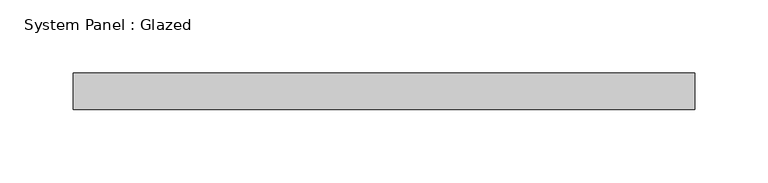
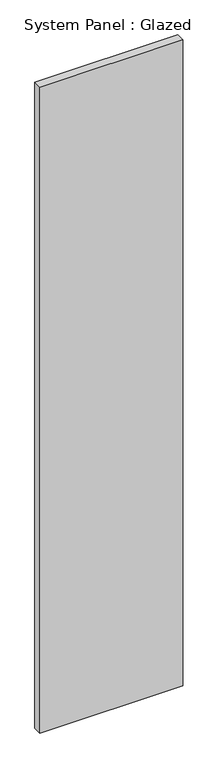
"""IFC4 building model written with IfcOpenShell, lengths in millimetres: plate geometry, System Panel : Glazed."""

from ifc_helpers import new_model, si_unit, origin, origin_with_axes, place, context, project, spatial, polyline, outline, extrude, source, transform, mapped, element, save


def system_panel_glazed_248dfa94(model_context):
    return source(origin(), model_context, "Body", "SweptSolid", [
        extrude(outline(polyline([(212.5000001, 24.5), (-212.5000001, 24.5), (-212.5000001, 49.5), (212.5000001, 49.5), (212.5000001, 24.5)])), origin_with_axes(), (0.0, 0.0, 1.0), 2030.4462072),
    ])


if __name__ == "__main__":
    model = new_model("IFC4")
    model_context = context("Model", 3, world=origin())
    ifc_project = project(units=[si_unit("LENGTHUNIT", "METRE", prefix="MILLI")], contexts=[model_context])
    site = spatial("IfcSite", under=ifc_project)
    building = spatial("IfcBuilding", under=site)
    placement = place(None, origin())
    system_panel_glazed_shape = system_panel_glazed_248dfa94(model_context)
    element("IfcPlate", 1, ObjectType="System Panel : Glazed", at=placement, inside=building, context=model_context, shape_type="MappedRepresentation", body=[
        mapped(system_panel_glazed_shape, transform((0.0, 0.0, 0.0), x_axis=(1.0, 0.0, 0.0), y_axis=(0.0, 1.0, 0.0), z_axis=(0.0, 0.0, 1.0))),
    ])
    save(model, "model.ifc")

# Revit data of these elements
# Type "System Panel : Glazed"
#   Construction Type Id = "GSP4R"
#   Analytic Construction = "1/8 in Pilkington single glazing"
#   Visual Light Transmittance = 0.9
#   Solar Heat Gain Coefficient = 0.86
#   Heat Transfer Coefficient (U) = 6.7069 W/(m²·K)
#   Define Thermal Properties by = 1
# Element 1 (IfcPlate, "System Panel : Glazed")
#   Materials on its faces: "Glass"
# Materials
#   "Glass": class "Glass", colour RGB 0 128 192, transparency 0.9, Description = "Soda Lime Glass", Cost = 0
